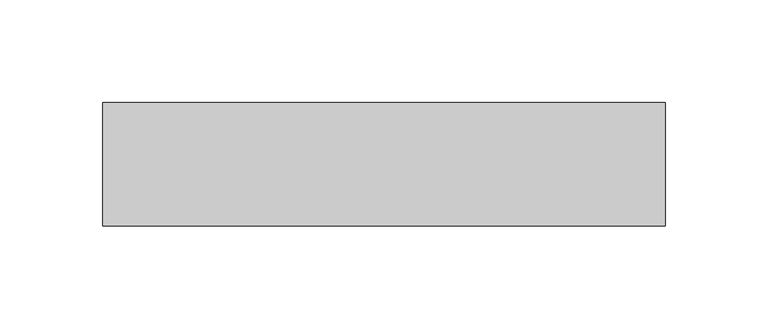
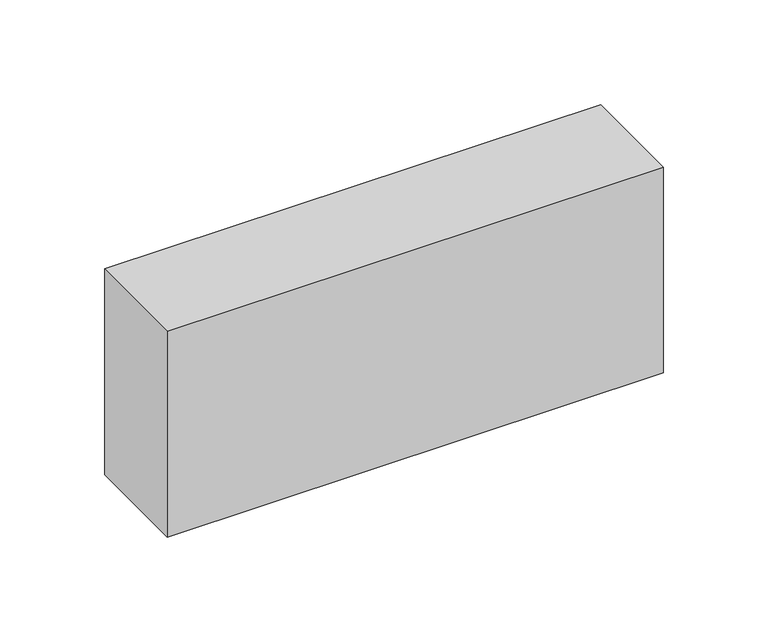
"""IFC4 building model written with IfcOpenShell, lengths in millimetres: beam geometry, Madeira de lei : Berço 6x12cm."""

import ifcopenshell
import ifcopenshell.guid

model = None  # the IFC model being written
_history = None  # IfcOwnerHistory: only IFC2X3 demands one
_inside = {}  # id of a spatial element -> (the spatial element, [elements in it])
_under = {}  # id of a project, library or spatial element -> (it, [spatial elements below it])
_declared = {}  # id of a project -> (the project, [libraries it declares])
_typed = {}  # id of a type object -> (the type object, [elements of that type])
_made_of = {}  # id of a material, layer set ... -> (it, [elements and type objects made of it])


def new_model(schema):
    """Start an empty IFC model of exactly this schema.

    Asked for "IFC4X3", IfcOpenShell would pick the latest addendum, in which some entities
    have other attributes; the version numbers below select the first issue.
    IFC2X3 requires an IfcOwnerHistory on every rooted entity: one is made here for all.
    """
    global model, _history
    if schema == "IFC4X3":
        model = ifcopenshell.file(schema_version=(4, 3, 0, 0))
    else:
        model = ifcopenshell.file(schema=schema)
    _inside.clear()
    _under.clear()
    _declared.clear()
    _typed.clear()
    _made_of.clear()
    _history = None
    if model.schema == "IFC2X3":
        org = make("IfcOrganization", Name="unknown")
        user = make(
            "IfcPersonAndOrganization",
            ThePerson=make("IfcPerson", FamilyName="unknown"),
            TheOrganization=org,
        )
        app = make(
            "IfcApplication",
            ApplicationDeveloper=org,
            Version="unknown",
            ApplicationFullName="unknown",
            ApplicationIdentifier="unknown",
        )
        _history = make(
            "IfcOwnerHistory",
            OwningUser=user,
            OwningApplication=app,
            ChangeAction="ADDED",
            CreationDate=0,
        )
    return model


def make(cls, **values):
    """One entity of the class cls with the attributes given. An attribute that is None is left unset."""
    return model.create_entity(
        cls, **{name: value for name, value in values.items() if value is not None}
    )


def rooted(cls, **values):
    """An entity with a GlobalId (a new one), such as an element, a storey or a relation."""
    return make(cls, GlobalId=ifcopenshell.guid.new(), OwnerHistory=_history, **values)


def si_unit(unit_type, name, prefix=None):
    """IfcSIUnit, for example si_unit("LENGTHUNIT", "METRE", prefix="MILLI")."""
    return make("IfcSIUnit", UnitType=unit_type, Prefix=prefix, Name=name)


def assignment(units):
    """IfcUnitAssignment: the units of a project."""
    return None if units is None else make("IfcUnitAssignment", Units=units)


def point(xyz):
    """IfcCartesianPoint."""
    return None if xyz is None else make("IfcCartesianPoint", Coordinates=xyz)


def direction(xyz):
    """IfcDirection."""
    return None if xyz is None else make("IfcDirection", DirectionRatios=xyz)


def frame(location, z_axis=None, x_axis=None):
    """IfcAxis2Placement3D, a coordinate frame: its origin and axes. An axis left out is left unset."""
    return make(
        "IfcAxis2Placement3D",
        Location=point(location),
        Axis=direction(z_axis),
        RefDirection=direction(x_axis),
    )


def origin():
    """The frame at (0, 0, 0) with its axes left unset."""
    return frame((0.0, 0.0, 0.0))


def place(relative_to, where):
    """IfcLocalPlacement: puts the frame where relative to a parent placement (None: the world)."""
    return make(
        "IfcLocalPlacement", PlacementRelTo=relative_to, RelativePlacement=where
    )


def context(
    kind, dimensions, precision=None, world=None, true_north=None, identifier=None
):
    """IfcGeometricRepresentationContext, for example the 3D "Model" context."""
    return make(
        "IfcGeometricRepresentationContext",
        ContextIdentifier=identifier,
        ContextType=kind,
        CoordinateSpaceDimension=dimensions,
        Precision=precision,
        WorldCoordinateSystem=world,
        TrueNorth=true_north,
    )


def project(units=None, contexts=None):
    """IfcProject with its units and contexts."""
    return rooted(
        "IfcProject",
        Name="project",
        RepresentationContexts=contexts,
        UnitsInContext=assignment(units),
    )


def spatial(cls, under=None, at=None, **own):
    """A site, building, storey or space (cls), placed at a placement, below another one or the project."""
    s = rooted(cls, ObjectPlacement=at, **own)
    if under is not None:
        _under.setdefault(under.id(), (under, []))[1].append(s)
    return s


def polyline(points):
    """IfcPolyline through the points."""
    return make("IfcPolyline", Points=[point(p) for p in points])


def outline(outer, holes=None, kind="AREA"):
    """IfcArbitraryClosedProfileDef: a profile drawn as a closed curve; with holes, ...WithVoids."""
    if holes is None:
        return make("IfcArbitraryClosedProfileDef", ProfileType=kind, OuterCurve=outer)
    return make(
        "IfcArbitraryProfileDefWithVoids",
        ProfileType=kind,
        OuterCurve=outer,
        InnerCurves=holes,
    )


def extrude(swept, where, along, depth):
    """IfcExtrudedAreaSolid: the profile swept, set in the frame where, extruded along a direction by depth."""
    return make(
        "IfcExtrudedAreaSolid",
        SweptArea=swept,
        Position=where,
        ExtrudedDirection=direction(along),
        Depth=depth,
    )


def shape(context_of_items, identifier, shape_type, items):
    """IfcShapeRepresentation: the items that make up one representation, for example the "Body"."""
    return make(
        "IfcShapeRepresentation",
        ContextOfItems=context_of_items,
        RepresentationIdentifier=identifier,
        RepresentationType=shape_type,
        Items=items,
    )


def source(mapping_origin, context_of_items, identifier, shape_type, items):
    """IfcRepresentationMap: a shape defined once, which mapped items show again and again."""
    return make(
        "IfcRepresentationMap",
        MappingOrigin=mapping_origin,
        MappedRepresentation=shape(context_of_items, identifier, shape_type, items),
    )


def transform(
    local_origin,
    x_axis=None,
    y_axis=None,
    z_axis=None,
    scale=None,
    scale2=None,
    scale3=None,
    uniform=True,
):
    """IfcCartesianTransformationOperator3D, or its non-uniform kind. x_axis, y_axis, z_axis: its Axis1, 2, 3."""
    if uniform:
        return make(
            "IfcCartesianTransformationOperator3D",
            Axis1=direction(x_axis),
            Axis2=direction(y_axis),
            LocalOrigin=point(local_origin),
            Scale=scale,
            Axis3=direction(z_axis),
        )
    return make(
        "IfcCartesianTransformationOperator3DnonUniform",
        Axis1=direction(x_axis),
        Axis2=direction(y_axis),
        LocalOrigin=point(local_origin),
        Scale=scale,
        Axis3=direction(z_axis),
        Scale2=scale2,
        Scale3=scale3,
    )


def mapped(mapping_source, mapping_target):
    """IfcMappedItem: shows the shape of a source again, moved by a transform."""
    return make(
        "IfcMappedItem", MappingSource=mapping_source, MappingTarget=mapping_target
    )


def made_of(thing, what):
    """Note that an element or type object is made of a material, layer set ...; save() writes the relation."""
    if what is not None:
        _made_of.setdefault(what.id(), (what, []))[1].append(thing)
    return thing


def element(
    cls,
    number,
    at=None,
    inside=None,
    cuts=None,
    type_object=None,
    material=None,
    context=None,
    identifier="Body",
    shape_type=None,
    held_by="IfcProductDefinitionShape",
    body=None,
    shapes=None,
    **own,
):
    """One element of the class cls, such as IfcWall. Its Tag is "e" and its number.

    at: its placement. inside: the storey or other place that contains it. cuts: it is an
    opening in that element (IfcRelVoidsElement). A single representation is given by context,
    identifier, shape_type and body (its items); several are given by shapes. held_by: the class
    of the entity that holds the representations. save() writes the other relations.
    """
    e = rooted(cls, Tag="e%d" % number, ObjectPlacement=at, **own)
    if body is not None:
        shapes = [shape(context, identifier, shape_type, body)]
    if shapes is not None:
        e.Representation = make(held_by, Representations=shapes)
    if inside is not None:
        _inside.setdefault(inside.id(), (inside, []))[1].append(e)
    if cuts is not None:
        rooted(
            "IfcRelVoidsElement", RelatingBuildingElement=cuts, RelatedOpeningElement=e
        )
    if type_object is not None:
        _typed.setdefault(type_object.id(), (type_object, []))[1].append(e)
    return made_of(e, material)


def aggregate(whole, parts):
    """IfcRelAggregates: a whole, such as a stair, and the parts it consists of."""
    return rooted("IfcRelAggregates", RelatingObject=whole, RelatedObjects=parts)


def save(model, path):
    """Write the relations noted so far, then the file.

    IfcRelAggregates (storeys below a building ...), IfcRelContainedInSpatialStructure (elements
    in a storey), IfcRelDefinesByType, IfcRelAssociatesMaterial and IfcRelDeclares: one each for
    every whole, place, type object, material and project.
    """
    for whole, parts in _under.values():
        aggregate(whole, parts)
    for where, things in _inside.values():
        rooted(
            "IfcRelContainedInSpatialStructure",
            RelatedElements=things,
            RelatingStructure=where,
        )
    for kind, things in _typed.values():
        rooted("IfcRelDefinesByType", RelatedObjects=things, RelatingType=kind)
    for what, things in _made_of.values():
        rooted("IfcRelAssociatesMaterial", RelatedObjects=things, RelatingMaterial=what)
    for by, libraries in _declared.values():
        rooted("IfcRelDeclares", RelatingContext=by, RelatedDefinitions=libraries)
    model.write(path)


def beam_88f0ebe1(model_context):
    return source(origin(), model_context, "Body", "SweptSolid", [
        extrude(outline(polyline([(136.7503096, 30.0), (136.7503096, -30.0), (-136.7503096, -30.0), (-136.7503096, 30.0), (136.7503096, 30.0)])), frame((0.0, 0.0, -60.0), z_axis=(0.0, 0.0, 1.0), x_axis=(1.0, 0.0, 0.0)), (0.0, 0.0, 1.0), 120.0),
    ])


if __name__ == "__main__":
    model = new_model("IFC4")
    model_context = context("Model", 3, world=origin())
    ifc_project = project(units=[si_unit("LENGTHUNIT", "METRE", prefix="MILLI")], contexts=[model_context])
    site = spatial("IfcSite", under=ifc_project)
    building = spatial("IfcBuilding", under=site)
    placement = place(None, origin())
    beam_shape = beam_88f0ebe1(model_context)
    element("IfcBeam", 1, ObjectType="Madeira de lei : Berço 6x12cm", at=placement, inside=building, context=model_context, shape_type="MappedRepresentation", body=[
        mapped(beam_shape, transform((0.0, 0.0, 0.0), x_axis=(1.0, 0.0, 0.0), y_axis=(0.0, 1.0, 0.0), z_axis=(0.0, 0.0, 1.0))),
    ])
    save(model, "model.ifc")

# Revit data of these elements
# Type "Madeira de lei : Berço 6x12cm"
#   A = 0.02 m²
#   Length [instance default] = 1.524 m
#   b = 0.06 m
#   d = 0.12 m
#   Structural Material [instance default] = none
#   Assembly Code = ""
# Element 1 (IfcBeam, "Madeira de lei : Berço 6x12cm")
#   Structural Material = .MADEIRAMENTO
#   Materials on its faces: ".MADEIRAMENTO"
# Materials
#   ".MADEIRAMENTO": class ".CC_MADEIRAS", colour RGB 212 179 113, transparency 0, Cost = 0
